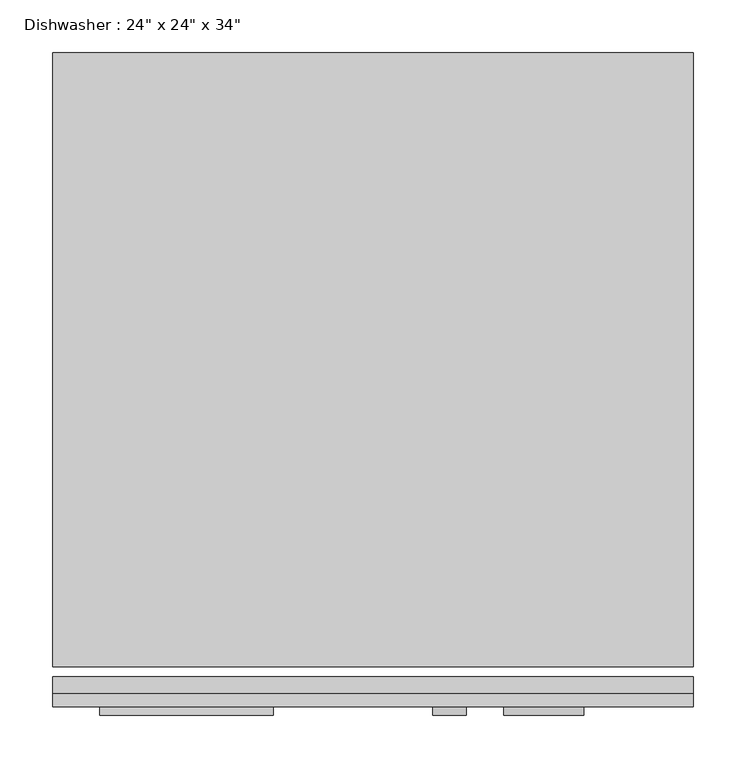
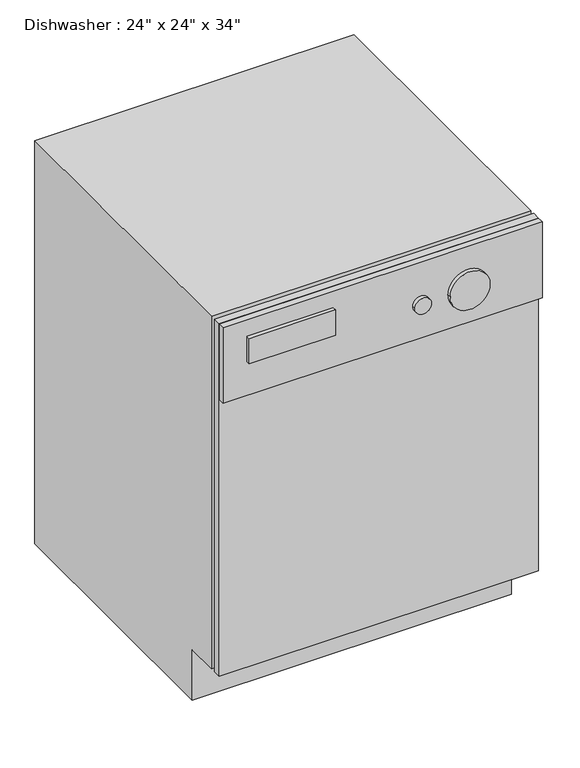
"""IFC4 building model written with IfcOpenShell, lengths in millimetres: proxy geometry."""

from ifc_helpers import new_model, si_unit, point, frame, frame_2d, origin, place, context, project, spatial, polyline, circle_curve, trimmed, segment, composite_curve, outline, extrude, source, transform, mapped, element, save


def proxy_603acf02(model_context):
    return source(origin(), model_context, "Body", "SweptSolid", [
        extrude(outline(polyline([(687.1174685, -38.3504352), (77.5174685, -38.3504352), (77.5174685, -22.4754352), (687.1174685, -22.4754352), (687.1174685, -38.3504352)])), frame((0.0, 0.0, 101.6), z_axis=(0.0, 0.0, 1.0), x_axis=(1.0, 0.0, 0.0)), (0.0, 0.0, 1.0), 711.2),
        extrude(outline(polyline([(687.1174685, -38.3504352), (687.1174685, -51.0504352), (77.5174685, -51.0504352), (77.5174685, -38.3504352), (687.1174685, -38.3504352)])), frame((0.0, 0.0, 660.4), z_axis=(0.0, 0.0, 1.0), x_axis=(1.0, 0.0, 0.0)), (0.0, 0.0, 1.0), 152.4),
        extrude(outline(polyline([(571.2495648, 0.0), (50.5495648, 0.0), (50.5495648, 101.6), (-12.9504352, 101.6), (-12.9504352, 812.8), (571.2495648, 812.8), (571.2495648, 0.0)])), frame((77.5174685, 0.0, 0.0), z_axis=(1.0, 0.0, 0.0), x_axis=(0.0, 1.0, 0.0)), (0.0, 0.0, 1.0), 609.6),
        extrude(outline(polyline([(287.6378068, -59.1863727), (122.5378068, -59.1863727), (122.5378068, -51.0504352), (287.6378068, -51.0504352), (287.6378068, -59.1863727)])), frame((0.0, 0.0, 729.2846419), z_axis=(0.0, 0.0, 1.0), x_axis=(1.0, 0.0, 0.0)), (0.0, 0.0, 1.0), 50.8),
        extrude(outline(composite_curve([segment(trimmed(circle_curve(frame_2d((729.2846419, 544.7247133)), 38.1), [point((729.2846419, 506.6247133))], [point((729.2846419, 582.8247133))], False, "CARTESIAN"), True, "CONTINUOUS"), segment(trimmed(circle_curve(frame_2d((729.2846419, 544.7247133)), 38.1), [point((729.2846419, 582.8247133))], [point((729.2846419, 506.6247133))], False, "CARTESIAN"), True, "CONTINUOUS")], self_intersect=False)), frame((0.0, -59.1863727, 0.0), z_axis=(0.0, 1.0, 0.0), x_axis=(0.0, 0.0, 1.0)), (0.0, 0.0, 1.0), 8.1359375),
        extrude(outline(composite_curve([segment(trimmed(circle_curve(frame_2d((729.2846419, 455.195318)), 15.875), [point((729.2846419, 439.320318))], [point((729.2846419, 471.070318))], False, "CARTESIAN"), True, "CONTINUOUS"), segment(trimmed(circle_curve(frame_2d((729.2846419, 455.195318)), 15.875), [point((729.2846419, 471.070318))], [point((729.2846419, 439.320318))], False, "CARTESIAN"), True, "CONTINUOUS")], self_intersect=False)), frame((0.0, -59.1863727, 0.0), z_axis=(0.0, 1.0, 0.0), x_axis=(0.0, 0.0, 1.0)), (0.0, 0.0, 1.0), 8.1359375),
    ])


if __name__ == "__main__":
    model = new_model("IFC4")
    model_context = context("Model", 3, world=origin())
    ifc_project = project(units=[si_unit("LENGTHUNIT", "METRE", prefix="MILLI")], contexts=[model_context])
    site = spatial("IfcSite", under=ifc_project)
    building = spatial("IfcBuilding", under=site)
    placement = place(None, origin())
    proxy_shape = proxy_603acf02(model_context)
    element("IfcBuildingElementProxy", 1, Name="Dishwasher : 24\" x 24\" x 34\"", ObjectType="Dishwasher : 24\" x 24\" x 34\"", at=placement, inside=building, context=model_context, shape_type="MappedRepresentation", body=[
        mapped(proxy_shape, transform((0.0, 0.0, 0.0), x_axis=(1.0, 0.0, 0.0), y_axis=(0.0, 1.0, 0.0), z_axis=(0.0, 0.0, 1.0))),
    ])
    save(model, "model.ifc")

# Revit data of these elements
# Type "Dishwasher : 24\" x 24\" x 34\""
#   Label = "DW"
#   Assembly Code = "E1090400"
#   Depth = 2' - 0"
#   Height = 2' - 8"
#   Width = 2' - 0"
#   Dishwasher Material = Metal - Paint Finish - Ivory,Glossy
#   Panel Face Material = Plastic - Black
# Element 1 (IfcBuildingElementProxy, "Dishwasher : 24\" x 24\" x 34\"")
#   Materials on its faces: "Speciality Equipment"
# Materials
#   "Metal - Paint Finish - Ivory,Glossy": class "Unassigned", colour RGB 247 247 239, transparency 0
#   "Plastic - Black": class "Plastic", colour RGB 0 0 0, transparency 0
#   "Speciality Equipment": class "Generic", colour RGB 255 255 255, transparency 0, Cost = 0
